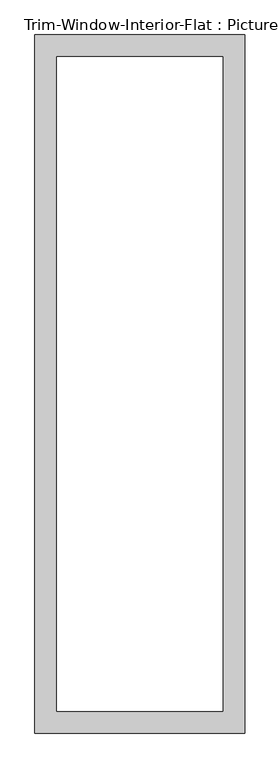
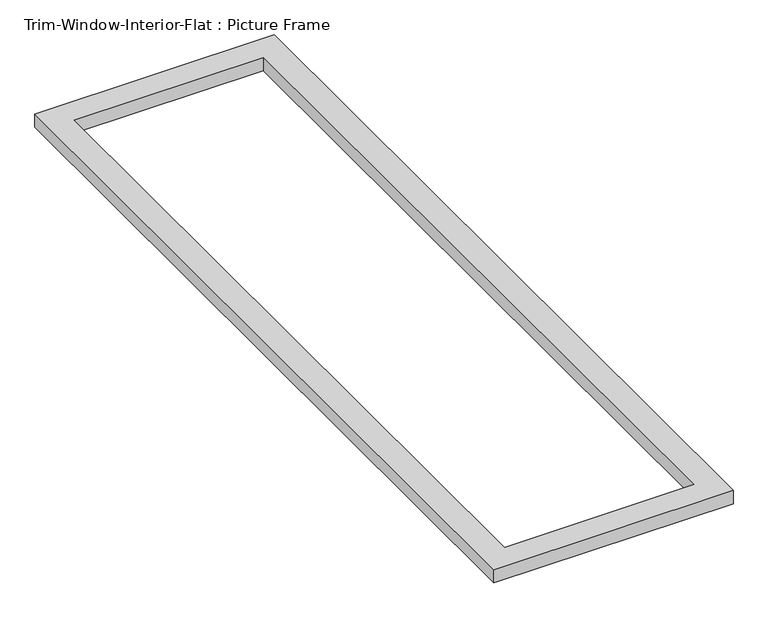
"""IFC4 building model written with IfcOpenShell, lengths in millimetres: proxy geometry, Trim-Window-Interior-Flat : Picture Frame."""

from ifc_helpers import new_model, si_unit, origin, origin_with_axes, place, context, project, spatial, polyline, outline, extrude, source, transform, mapped, element, save


def trim_window_interior_flat_picture_frame_db28ea87(model_context):
    return source(origin(), model_context, "Body", "SweptSolid", [
        extrude(outline(polyline([(273.05, 44.45), (273.05, -1771.65), (-273.05, -1771.65), (-273.05, 44.45), (273.05, 44.45)]), holes=[polyline([(215.9, -12.7), (-215.9, -12.7), (-215.9, -1714.5), (215.9, -1714.5), (215.9, -12.7)])]), origin_with_axes(), (0.0, 0.0, 1.0), 31.75),
    ])


if __name__ == "__main__":
    model = new_model("IFC4")
    model_context = context("Model", 3, world=origin())
    ifc_project = project(units=[si_unit("LENGTHUNIT", "METRE", prefix="MILLI")], contexts=[model_context])
    site = spatial("IfcSite", under=ifc_project)
    building = spatial("IfcBuilding", under=site)
    placement = place(None, origin())
    trim_window_interior_flat_picture_frame_shape = trim_window_interior_flat_picture_frame_db28ea87(model_context)
    element("IfcBuildingElementProxy", 1, Name="Trim-Window-Interior-Flat : Picture Frame", ObjectType="Trim-Window-Interior-Flat : Picture Frame", at=placement, inside=building, context=model_context, shape_type="MappedRepresentation", body=[
        mapped(trim_window_interior_flat_picture_frame_shape, transform((0.0, 0.0, 0.0), x_axis=(1.0, 0.0, 0.0), y_axis=(0.0, 1.0, 0.0), z_axis=(0.0, 0.0, 1.0))),
    ])
    save(model, "model.ifc")

# Revit data of these elements
# Type "Trim-Window-Interior-Flat : Picture Frame"
#   Trim Thickness_Picture Frame = 0' - 1 1/4"
#   Trim Width = 0' - 2 1/4"
#   Trim Thickness_with Sill = 0' - 0 3/4"
#   Sill Thickness = 0' - 1 1/4"
#   Opening Width [instance default] = 2' - 0"
#   Opening Height [instance default] = 3' - 0"
#   Default Elevation = 4' - 0"
#   Sill = no
#   Picture Frame = yes
#   Trim Material [instance default] = none
# Element 1 (IfcBuildingElementProxy, "Trim-Window-Interior-Flat : Picture Frame")
#   Opening Width = 1' - 6"
#   Opening Height = 5' - 8"
#   Trim Material = Wood - Stained
#   Materials on its faces: "Wood - Stained"
# Materials
#   "Wood - Stained": class "Wood", colour RGB 224 178 126, transparency 0, Cost = 0
